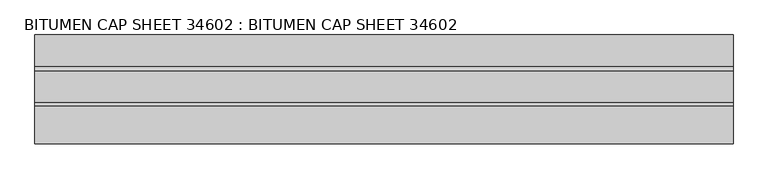
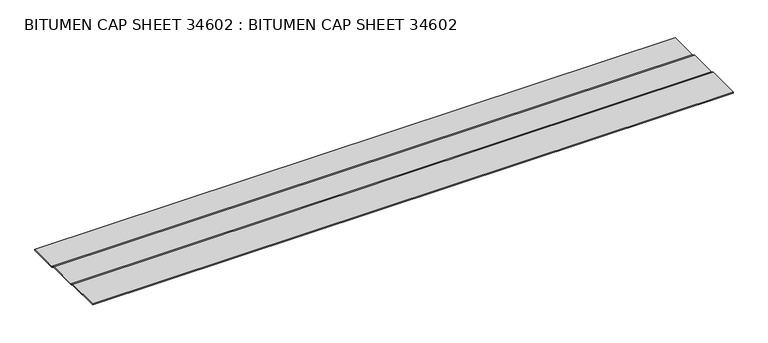
"""IFC4 building model written with IfcOpenShell, lengths in millimetres: proxy geometry, BITUMEN CAP SHEET 34602 : BITUMEN CAP SHEET 34602."""

import ifcopenshell
import ifcopenshell.guid

model = None  # the IFC model being written
_history = None  # IfcOwnerHistory: only IFC2X3 demands one
_inside = {}  # id of a spatial element -> (the spatial element, [elements in it])
_under = {}  # id of a project, library or spatial element -> (it, [spatial elements below it])
_declared = {}  # id of a project -> (the project, [libraries it declares])
_typed = {}  # id of a type object -> (the type object, [elements of that type])
_made_of = {}  # id of a material, layer set ... -> (it, [elements and type objects made of it])


def new_model(schema):
    """Start an empty IFC model of exactly this schema.

    Asked for "IFC4X3", IfcOpenShell would pick the latest addendum, in which some entities
    have other attributes; the version numbers below select the first issue.
    IFC2X3 requires an IfcOwnerHistory on every rooted entity: one is made here for all.
    """
    global model, _history
    if schema == "IFC4X3":
        model = ifcopenshell.file(schema_version=(4, 3, 0, 0))
    else:
        model = ifcopenshell.file(schema=schema)
    _inside.clear()
    _under.clear()
    _declared.clear()
    _typed.clear()
    _made_of.clear()
    _history = None
    if model.schema == "IFC2X3":
        org = make("IfcOrganization", Name="unknown")
        user = make(
            "IfcPersonAndOrganization",
            ThePerson=make("IfcPerson", FamilyName="unknown"),
            TheOrganization=org,
        )
        app = make(
            "IfcApplication",
            ApplicationDeveloper=org,
            Version="unknown",
            ApplicationFullName="unknown",
            ApplicationIdentifier="unknown",
        )
        _history = make(
            "IfcOwnerHistory",
            OwningUser=user,
            OwningApplication=app,
            ChangeAction="ADDED",
            CreationDate=0,
        )
    return model


def make(cls, **values):
    """One entity of the class cls with the attributes given. An attribute that is None is left unset."""
    return model.create_entity(
        cls, **{name: value for name, value in values.items() if value is not None}
    )


def rooted(cls, **values):
    """An entity with a GlobalId (a new one), such as an element, a storey or a relation."""
    return make(cls, GlobalId=ifcopenshell.guid.new(), OwnerHistory=_history, **values)


def si_unit(unit_type, name, prefix=None):
    """IfcSIUnit, for example si_unit("LENGTHUNIT", "METRE", prefix="MILLI")."""
    return make("IfcSIUnit", UnitType=unit_type, Prefix=prefix, Name=name)


def assignment(units):
    """IfcUnitAssignment: the units of a project."""
    return None if units is None else make("IfcUnitAssignment", Units=units)


def point(xyz):
    """IfcCartesianPoint."""
    return None if xyz is None else make("IfcCartesianPoint", Coordinates=xyz)


def direction(xyz):
    """IfcDirection."""
    return None if xyz is None else make("IfcDirection", DirectionRatios=xyz)


def frame(location, z_axis=None, x_axis=None):
    """IfcAxis2Placement3D, a coordinate frame: its origin and axes. An axis left out is left unset."""
    return make(
        "IfcAxis2Placement3D",
        Location=point(location),
        Axis=direction(z_axis),
        RefDirection=direction(x_axis),
    )


def origin():
    """The frame at (0, 0, 0) with its axes left unset."""
    return frame((0.0, 0.0, 0.0))


def place(relative_to, where):
    """IfcLocalPlacement: puts the frame where relative to a parent placement (None: the world)."""
    return make(
        "IfcLocalPlacement", PlacementRelTo=relative_to, RelativePlacement=where
    )


def context(
    kind, dimensions, precision=None, world=None, true_north=None, identifier=None
):
    """IfcGeometricRepresentationContext, for example the 3D "Model" context."""
    return make(
        "IfcGeometricRepresentationContext",
        ContextIdentifier=identifier,
        ContextType=kind,
        CoordinateSpaceDimension=dimensions,
        Precision=precision,
        WorldCoordinateSystem=world,
        TrueNorth=true_north,
    )


def project(units=None, contexts=None):
    """IfcProject with its units and contexts."""
    return rooted(
        "IfcProject",
        Name="project",
        RepresentationContexts=contexts,
        UnitsInContext=assignment(units),
    )


def spatial(cls, under=None, at=None, **own):
    """A site, building, storey or space (cls), placed at a placement, below another one or the project."""
    s = rooted(cls, ObjectPlacement=at, **own)
    if under is not None:
        _under.setdefault(under.id(), (under, []))[1].append(s)
    return s


def polyline(points):
    """IfcPolyline through the points."""
    return make("IfcPolyline", Points=[point(p) for p in points])


def outline(outer, holes=None, kind="AREA"):
    """IfcArbitraryClosedProfileDef: a profile drawn as a closed curve; with holes, ...WithVoids."""
    if holes is None:
        return make("IfcArbitraryClosedProfileDef", ProfileType=kind, OuterCurve=outer)
    return make(
        "IfcArbitraryProfileDefWithVoids",
        ProfileType=kind,
        OuterCurve=outer,
        InnerCurves=holes,
    )


def extrude(swept, where, along, depth):
    """IfcExtrudedAreaSolid: the profile swept, set in the frame where, extruded along a direction by depth."""
    return make(
        "IfcExtrudedAreaSolid",
        SweptArea=swept,
        Position=where,
        ExtrudedDirection=direction(along),
        Depth=depth,
    )


def shape(context_of_items, identifier, shape_type, items):
    """IfcShapeRepresentation: the items that make up one representation, for example the "Body"."""
    return make(
        "IfcShapeRepresentation",
        ContextOfItems=context_of_items,
        RepresentationIdentifier=identifier,
        RepresentationType=shape_type,
        Items=items,
    )


def source(mapping_origin, context_of_items, identifier, shape_type, items):
    """IfcRepresentationMap: a shape defined once, which mapped items show again and again."""
    return make(
        "IfcRepresentationMap",
        MappingOrigin=mapping_origin,
        MappedRepresentation=shape(context_of_items, identifier, shape_type, items),
    )


def transform(
    local_origin,
    x_axis=None,
    y_axis=None,
    z_axis=None,
    scale=None,
    scale2=None,
    scale3=None,
    uniform=True,
):
    """IfcCartesianTransformationOperator3D, or its non-uniform kind. x_axis, y_axis, z_axis: its Axis1, 2, 3."""
    if uniform:
        return make(
            "IfcCartesianTransformationOperator3D",
            Axis1=direction(x_axis),
            Axis2=direction(y_axis),
            LocalOrigin=point(local_origin),
            Scale=scale,
            Axis3=direction(z_axis),
        )
    return make(
        "IfcCartesianTransformationOperator3DnonUniform",
        Axis1=direction(x_axis),
        Axis2=direction(y_axis),
        LocalOrigin=point(local_origin),
        Scale=scale,
        Axis3=direction(z_axis),
        Scale2=scale2,
        Scale3=scale3,
    )


def mapped(mapping_source, mapping_target):
    """IfcMappedItem: shows the shape of a source again, moved by a transform."""
    return make(
        "IfcMappedItem", MappingSource=mapping_source, MappingTarget=mapping_target
    )


def made_of(thing, what):
    """Note that an element or type object is made of a material, layer set ...; save() writes the relation."""
    if what is not None:
        _made_of.setdefault(what.id(), (what, []))[1].append(thing)
    return thing


def element(
    cls,
    number,
    at=None,
    inside=None,
    cuts=None,
    type_object=None,
    material=None,
    context=None,
    identifier="Body",
    shape_type=None,
    held_by="IfcProductDefinitionShape",
    body=None,
    shapes=None,
    **own,
):
    """One element of the class cls, such as IfcWall. Its Tag is "e" and its number.

    at: its placement. inside: the storey or other place that contains it. cuts: it is an
    opening in that element (IfcRelVoidsElement). A single representation is given by context,
    identifier, shape_type and body (its items); several are given by shapes. held_by: the class
    of the entity that holds the representations. save() writes the other relations.
    """
    e = rooted(cls, Tag="e%d" % number, ObjectPlacement=at, **own)
    if body is not None:
        shapes = [shape(context, identifier, shape_type, body)]
    if shapes is not None:
        e.Representation = make(held_by, Representations=shapes)
    if inside is not None:
        _inside.setdefault(inside.id(), (inside, []))[1].append(e)
    if cuts is not None:
        rooted(
            "IfcRelVoidsElement", RelatingBuildingElement=cuts, RelatedOpeningElement=e
        )
    if type_object is not None:
        _typed.setdefault(type_object.id(), (type_object, []))[1].append(e)
    return made_of(e, material)


def aggregate(whole, parts):
    """IfcRelAggregates: a whole, such as a stair, and the parts it consists of."""
    return rooted("IfcRelAggregates", RelatingObject=whole, RelatedObjects=parts)


def save(model, path):
    """Write the relations noted so far, then the file.

    IfcRelAggregates (storeys below a building ...), IfcRelContainedInSpatialStructure (elements
    in a storey), IfcRelDefinesByType, IfcRelAssociatesMaterial and IfcRelDeclares: one each for
    every whole, place, type object, material and project.
    """
    for whole, parts in _under.values():
        aggregate(whole, parts)
    for where, things in _inside.values():
        rooted(
            "IfcRelContainedInSpatialStructure",
            RelatedElements=things,
            RelatingStructure=where,
        )
    for kind, things in _typed.values():
        rooted("IfcRelDefinesByType", RelatedObjects=things, RelatingType=kind)
    for what, things in _made_of.values():
        rooted("IfcRelAssociatesMaterial", RelatedObjects=things, RelatingMaterial=what)
    for by, libraries in _declared.values():
        rooted("IfcRelDeclares", RelatingContext=by, RelatedDefinitions=libraries)
    model.write(path)


def bitumen_cap_sheet_34602_bitumen_cap_sheet_34602_a55ad838(model_context):
    return source(origin(), model_context, "Body", "SweptSolid", [
        extrude(outline(polyline([(-5237.2758356, 40238.7580714), (-5329.4404972, 40238.7580714), (-5341.9053158, 40244.0440809), (-5432.619472, 40244.0440809), (-5442.3358585, 40248.3766459), (-5549.5470696, 40248.3766459), (-5549.5470696, 40251.5518755), (-5441.660573, 40251.5518755), (-5431.9436715, 40247.2190809), (-5341.2599159, 40247.2190809), (-5328.7950972, 40241.9330714), (-5237.2758356, 40241.9330714), (-5237.2758356, 40238.7580714)])), frame((12382.7678845, 0.0, 0.0), z_axis=(1.0, 0.0, 0.0), x_axis=(0.0, 1.0, 0.0)), (0.0, 0.0, 1.0), 2000.25),
    ])


if __name__ == "__main__":
    model = new_model("IFC4")
    model_context = context("Model", 3, world=origin())
    ifc_project = project(units=[si_unit("LENGTHUNIT", "METRE", prefix="MILLI")], contexts=[model_context])
    site = spatial("IfcSite", under=ifc_project)
    building = spatial("IfcBuilding", under=site)
    placement = place(None, origin())
    bitumen_cap_sheet_34602_bitumen_cap_sheet_34602_shape = bitumen_cap_sheet_34602_bitumen_cap_sheet_34602_a55ad838(model_context)
    element("IfcBuildingElementProxy", 1, Name="BITUMEN CAP SHEET 34602 : BITUMEN CAP SHEET 34602", ObjectType="BITUMEN CAP SHEET 34602 : BITUMEN CAP SHEET 34602", at=placement, inside=building, context=model_context, shape_type="MappedRepresentation", body=[
        mapped(bitumen_cap_sheet_34602_bitumen_cap_sheet_34602_shape, transform((0.0, 0.0, 0.0), x_axis=(1.0, 0.0, 0.0), y_axis=(0.0, 1.0, 0.0), z_axis=(0.0, 0.0, 1.0))),
    ])
    save(model, "model.ifc")

# Revit data of these elements
# Type "BITUMEN CAP SHEET 34602 : BITUMEN CAP SHEET 34602"
#   NameOverride = "BITUMEN CAP SHEET"
# Element 1 (IfcBuildingElementProxy, "BITUMEN CAP SHEET 34602 : BITUMEN CAP SHEET 34602")
#   Materials on its faces: "MODIFIED BITUMEN GRANULE SURFACED CAP SHEET"
# Materials
#   "MODIFIED BITUMEN GRANULE SURFACED CAP SHEET": class "Unassigned", colour RGB 85 85 127, transparency 0
